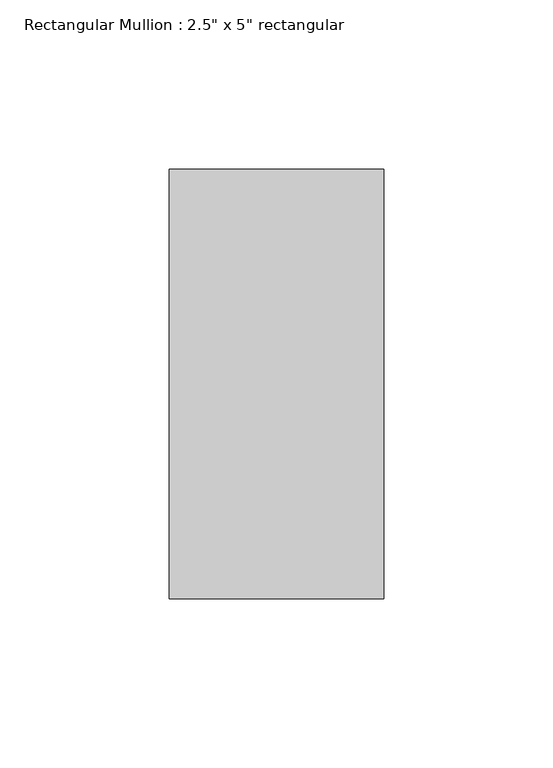
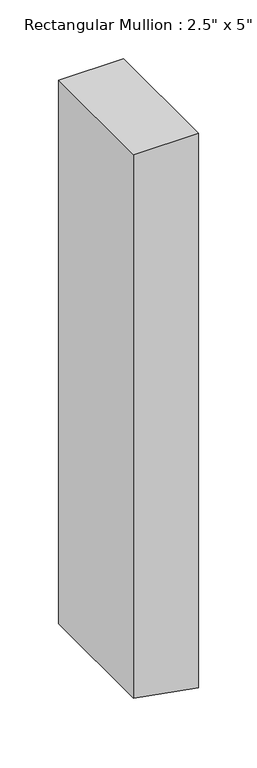
"""IFC4 building model written with IfcOpenShell, lengths in millimetres: member geometry."""

from ifc_helpers import new_model, si_unit, frame, origin, place, context, project, spatial, polyline, outline, extrude, source, transform, mapped, element, save


def member_0f56cb23(model_context):
    return source(origin(), model_context, "Body", "SweptSolid", [
        extrude(outline(polyline([(0.0, 31.75), (0.0, -31.75), (-563.2916809, -31.75), (-570.8343601, 11.0266593), (-574.4884442, 31.75), (0.0, 31.75)])), frame((0.0, -63.5, 0.0), z_axis=(0.0, 1.0, 0.0), x_axis=(0.0, 0.0, 1.0)), (0.0, 0.0, 1.0), 127.0),
    ])


if __name__ == "__main__":
    model = new_model("IFC4")
    model_context = context("Model", 3, world=origin())
    ifc_project = project(units=[si_unit("LENGTHUNIT", "METRE", prefix="MILLI")], contexts=[model_context])
    site = spatial("IfcSite", under=ifc_project)
    building = spatial("IfcBuilding", under=site)
    placement = place(None, origin())
    member_shape = member_0f56cb23(model_context)
    element("IfcMember", 1, ObjectType="Rectangular Mullion : 2.5\" x 5\" rectangular", at=placement, inside=building, context=model_context, shape_type="MappedRepresentation", body=[
        mapped(member_shape, transform((0.0, 0.0, 0.0), x_axis=(1.0, 0.0, 0.0), y_axis=(0.0, 1.0, 0.0), z_axis=(0.0, 0.0, 1.0))),
    ])
    save(model, "model.ifc")

# Revit data of these elements
# Type "Rectangular Mullion : 2.5\" x 5\" rectangular"
#   built-in parameter 1007304 = 0.416667 (stored number, unit not read)
#   built-in parameter 1007301 = 0.104167 (stored number, unit not read)
#   built-in parameter 1007300 = 0.104167 (stored number, unit not read)
# Element 1 (IfcMember, "Rectangular Mullion : 2.5\" x 5\" rectangular")
#   Materials on its faces: "Black Mullions"
# Materials
#   "Black Mullions": class "Wood", colour RGB 0 0 0, transparency 0, Cost = 0
